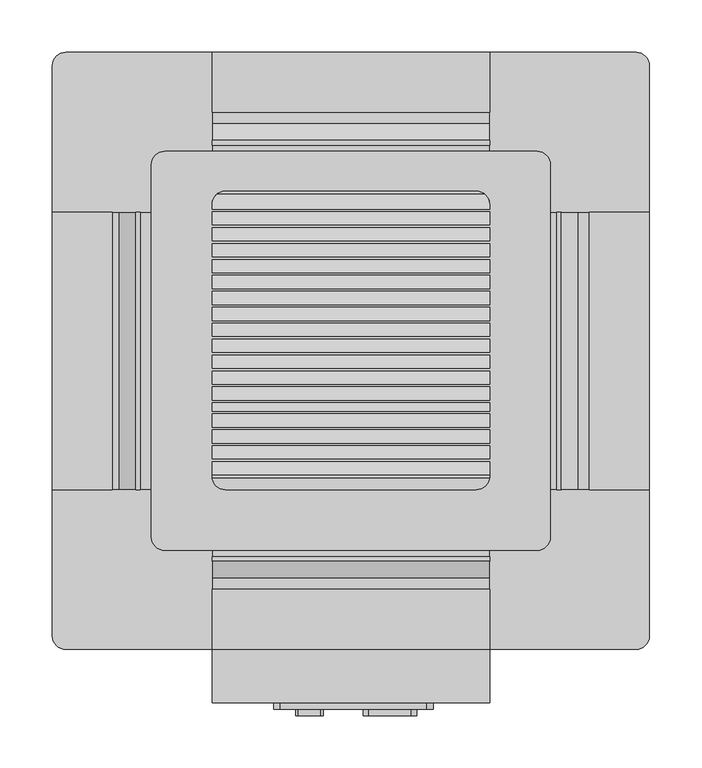
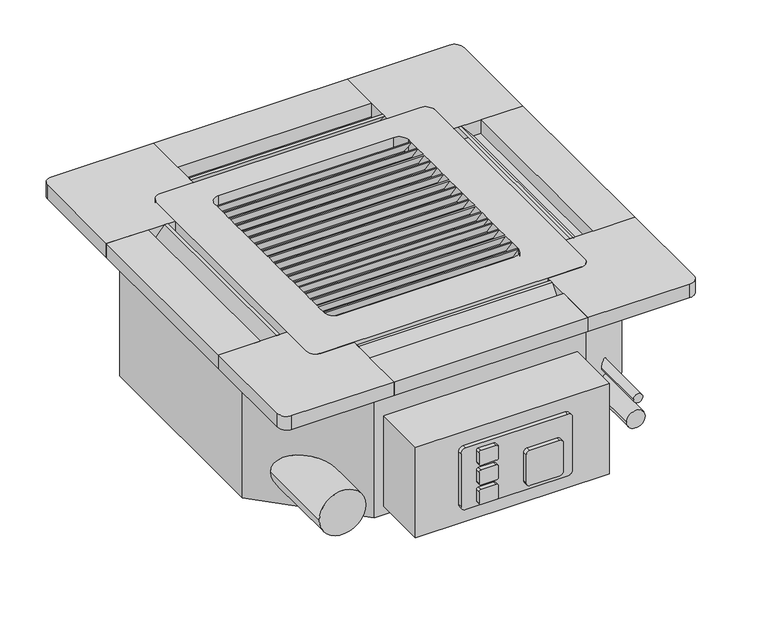
"""IFC4 building model written with IfcOpenShell, lengths in millimetres: proxy geometry, PLFY-P-NCMU-E_4-way_24x24 : PLFY-P12NCMU-E."""

import ifcopenshell
import ifcopenshell.guid

model = None  # the IFC model being written
_history = None  # IfcOwnerHistory: only IFC2X3 demands one
_inside = {}  # id of a spatial element -> (the spatial element, [elements in it])
_under = {}  # id of a project, library or spatial element -> (it, [spatial elements below it])
_declared = {}  # id of a project -> (the project, [libraries it declares])
_typed = {}  # id of a type object -> (the type object, [elements of that type])
_made_of = {}  # id of a material, layer set ... -> (it, [elements and type objects made of it])


def new_model(schema):
    """Start an empty IFC model of exactly this schema.

    Asked for "IFC4X3", IfcOpenShell would pick the latest addendum, in which some entities
    have other attributes; the version numbers below select the first issue.
    IFC2X3 requires an IfcOwnerHistory on every rooted entity: one is made here for all.
    """
    global model, _history
    if schema == "IFC4X3":
        model = ifcopenshell.file(schema_version=(4, 3, 0, 0))
    else:
        model = ifcopenshell.file(schema=schema)
    _inside.clear()
    _under.clear()
    _declared.clear()
    _typed.clear()
    _made_of.clear()
    _history = None
    if model.schema == "IFC2X3":
        org = make("IfcOrganization", Name="unknown")
        user = make(
            "IfcPersonAndOrganization",
            ThePerson=make("IfcPerson", FamilyName="unknown"),
            TheOrganization=org,
        )
        app = make(
            "IfcApplication",
            ApplicationDeveloper=org,
            Version="unknown",
            ApplicationFullName="unknown",
            ApplicationIdentifier="unknown",
        )
        _history = make(
            "IfcOwnerHistory",
            OwningUser=user,
            OwningApplication=app,
            ChangeAction="ADDED",
            CreationDate=0,
        )
    return model


def make(cls, **values):
    """One entity of the class cls with the attributes given. An attribute that is None is left unset."""
    return model.create_entity(
        cls, **{name: value for name, value in values.items() if value is not None}
    )


def rooted(cls, **values):
    """An entity with a GlobalId (a new one), such as an element, a storey or a relation."""
    return make(cls, GlobalId=ifcopenshell.guid.new(), OwnerHistory=_history, **values)


def si_unit(unit_type, name, prefix=None):
    """IfcSIUnit, for example si_unit("LENGTHUNIT", "METRE", prefix="MILLI")."""
    return make("IfcSIUnit", UnitType=unit_type, Prefix=prefix, Name=name)


def assignment(units):
    """IfcUnitAssignment: the units of a project."""
    return None if units is None else make("IfcUnitAssignment", Units=units)


def point(xyz):
    """IfcCartesianPoint."""
    return None if xyz is None else make("IfcCartesianPoint", Coordinates=xyz)


def direction(xyz):
    """IfcDirection."""
    return None if xyz is None else make("IfcDirection", DirectionRatios=xyz)


def frame(location, z_axis=None, x_axis=None):
    """IfcAxis2Placement3D, a coordinate frame: its origin and axes. An axis left out is left unset."""
    return make(
        "IfcAxis2Placement3D",
        Location=point(location),
        Axis=direction(z_axis),
        RefDirection=direction(x_axis),
    )


def frame_2d(location, x_axis=None):
    """IfcAxis2Placement2D, a coordinate frame in the plane: its origin and x axis."""
    return make(
        "IfcAxis2Placement2D", Location=point(location), RefDirection=direction(x_axis)
    )


def origin():
    """The frame at (0, 0, 0) with its axes left unset."""
    return frame((0.0, 0.0, 0.0))


def place(relative_to, where):
    """IfcLocalPlacement: puts the frame where relative to a parent placement (None: the world)."""
    return make(
        "IfcLocalPlacement", PlacementRelTo=relative_to, RelativePlacement=where
    )


def context(
    kind, dimensions, precision=None, world=None, true_north=None, identifier=None
):
    """IfcGeometricRepresentationContext, for example the 3D "Model" context."""
    return make(
        "IfcGeometricRepresentationContext",
        ContextIdentifier=identifier,
        ContextType=kind,
        CoordinateSpaceDimension=dimensions,
        Precision=precision,
        WorldCoordinateSystem=world,
        TrueNorth=true_north,
    )


def project(units=None, contexts=None):
    """IfcProject with its units and contexts."""
    return rooted(
        "IfcProject",
        Name="project",
        RepresentationContexts=contexts,
        UnitsInContext=assignment(units),
    )


def spatial(cls, under=None, at=None, **own):
    """A site, building, storey or space (cls), placed at a placement, below another one or the project."""
    s = rooted(cls, ObjectPlacement=at, **own)
    if under is not None:
        _under.setdefault(under.id(), (under, []))[1].append(s)
    return s


def polyline(points):
    """IfcPolyline through the points."""
    return make("IfcPolyline", Points=[point(p) for p in points])


def circle_curve(where, radius):
    """IfcCircle in the frame where."""
    return make("IfcCircle", Position=where, Radius=radius)


def ellipse_curve(where, semi_axis1, semi_axis2):
    """IfcEllipse in the frame where."""
    return make(
        "IfcEllipse", Position=where, SemiAxis1=semi_axis1, SemiAxis2=semi_axis2
    )


def trimmed(basis, trim1, trim2, sense, master):
    """IfcTrimmedCurve: the piece of a basis curve between two trims."""
    return make(
        "IfcTrimmedCurve",
        BasisCurve=basis,
        Trim1=trim1,
        Trim2=trim2,
        SenseAgreement=sense,
        MasterRepresentation=master,
    )


def segment(curve, same_sense, transition):
    """IfcCompositeCurveSegment."""
    return make(
        "IfcCompositeCurveSegment",
        Transition=transition,
        SameSense=same_sense,
        ParentCurve=curve,
    )


def composite_curve(segments, self_intersect=None):
    """IfcCompositeCurve: segments joined end to end."""
    return make("IfcCompositeCurve", Segments=segments, SelfIntersect=self_intersect)


def outline(outer, holes=None, kind="AREA"):
    """IfcArbitraryClosedProfileDef: a profile drawn as a closed curve; with holes, ...WithVoids."""
    if holes is None:
        return make("IfcArbitraryClosedProfileDef", ProfileType=kind, OuterCurve=outer)
    return make(
        "IfcArbitraryProfileDefWithVoids",
        ProfileType=kind,
        OuterCurve=outer,
        InnerCurves=holes,
    )


def extrude(swept, where, along, depth):
    """IfcExtrudedAreaSolid: the profile swept, set in the frame where, extruded along a direction by depth."""
    return make(
        "IfcExtrudedAreaSolid",
        SweptArea=swept,
        Position=where,
        ExtrudedDirection=direction(along),
        Depth=depth,
    )


def shape(context_of_items, identifier, shape_type, items):
    """IfcShapeRepresentation: the items that make up one representation, for example the "Body"."""
    return make(
        "IfcShapeRepresentation",
        ContextOfItems=context_of_items,
        RepresentationIdentifier=identifier,
        RepresentationType=shape_type,
        Items=items,
    )


def source(mapping_origin, context_of_items, identifier, shape_type, items):
    """IfcRepresentationMap: a shape defined once, which mapped items show again and again."""
    return make(
        "IfcRepresentationMap",
        MappingOrigin=mapping_origin,
        MappedRepresentation=shape(context_of_items, identifier, shape_type, items),
    )


def transform(
    local_origin,
    x_axis=None,
    y_axis=None,
    z_axis=None,
    scale=None,
    scale2=None,
    scale3=None,
    uniform=True,
):
    """IfcCartesianTransformationOperator3D, or its non-uniform kind. x_axis, y_axis, z_axis: its Axis1, 2, 3."""
    if uniform:
        return make(
            "IfcCartesianTransformationOperator3D",
            Axis1=direction(x_axis),
            Axis2=direction(y_axis),
            LocalOrigin=point(local_origin),
            Scale=scale,
            Axis3=direction(z_axis),
        )
    return make(
        "IfcCartesianTransformationOperator3DnonUniform",
        Axis1=direction(x_axis),
        Axis2=direction(y_axis),
        LocalOrigin=point(local_origin),
        Scale=scale,
        Axis3=direction(z_axis),
        Scale2=scale2,
        Scale3=scale3,
    )


def mapped(mapping_source, mapping_target):
    """IfcMappedItem: shows the shape of a source again, moved by a transform."""
    return make(
        "IfcMappedItem", MappingSource=mapping_source, MappingTarget=mapping_target
    )


def made_of(thing, what):
    """Note that an element or type object is made of a material, layer set ...; save() writes the relation."""
    if what is not None:
        _made_of.setdefault(what.id(), (what, []))[1].append(thing)
    return thing


def element(
    cls,
    number,
    at=None,
    inside=None,
    cuts=None,
    type_object=None,
    material=None,
    context=None,
    identifier="Body",
    shape_type=None,
    held_by="IfcProductDefinitionShape",
    body=None,
    shapes=None,
    **own,
):
    """One element of the class cls, such as IfcWall. Its Tag is "e" and its number.

    at: its placement. inside: the storey or other place that contains it. cuts: it is an
    opening in that element (IfcRelVoidsElement). A single representation is given by context,
    identifier, shape_type and body (its items); several are given by shapes. held_by: the class
    of the entity that holds the representations. save() writes the other relations.
    """
    e = rooted(cls, Tag="e%d" % number, ObjectPlacement=at, **own)
    if body is not None:
        shapes = [shape(context, identifier, shape_type, body)]
    if shapes is not None:
        e.Representation = make(held_by, Representations=shapes)
    if inside is not None:
        _inside.setdefault(inside.id(), (inside, []))[1].append(e)
    if cuts is not None:
        rooted(
            "IfcRelVoidsElement", RelatingBuildingElement=cuts, RelatedOpeningElement=e
        )
    if type_object is not None:
        _typed.setdefault(type_object.id(), (type_object, []))[1].append(e)
    return made_of(e, material)


def aggregate(whole, parts):
    """IfcRelAggregates: a whole, such as a stair, and the parts it consists of."""
    return rooted("IfcRelAggregates", RelatingObject=whole, RelatedObjects=parts)


def save(model, path):
    """Write the relations noted so far, then the file.

    IfcRelAggregates (storeys below a building ...), IfcRelContainedInSpatialStructure (elements
    in a storey), IfcRelDefinesByType, IfcRelAssociatesMaterial and IfcRelDeclares: one each for
    every whole, place, type object, material and project.
    """
    for whole, parts in _under.values():
        aggregate(whole, parts)
    for where, things in _inside.values():
        rooted(
            "IfcRelContainedInSpatialStructure",
            RelatedElements=things,
            RelatingStructure=where,
        )
    for kind, things in _typed.values():
        rooted("IfcRelDefinesByType", RelatedObjects=things, RelatingType=kind)
    for what, things in _made_of.values():
        rooted("IfcRelAssociatesMaterial", RelatedObjects=things, RelatingMaterial=what)
    for by, libraries in _declared.values():
        rooted("IfcRelDeclares", RelatingContext=by, RelatedDefinitions=libraries)
    model.write(path)


def plane_surface(at):
    """IfcPlane: the flat surface through the origin of the frame at, square to its z axis."""
    return make("IfcPlane", Position=at)


def cylinder_surface(at, radius):
    """IfcCylindricalSurface: all points at the distance radius from the z axis of the frame at."""
    return make("IfcCylindricalSurface", Position=at, Radius=radius)


def revolved_surface(curve, axis_point, axis_direction):
    """IfcSurfaceOfRevolution: the curve turned about the line through axis_point along axis_direction."""
    return make(
        "IfcSurfaceOfRevolution",
        SweptCurve=make("IfcArbitraryOpenProfileDef", ProfileType="CURVE", Curve=curve),
        AxisPosition=make("IfcAxis1Placement", Location=point(axis_point), Axis=direction(axis_direction)),
    )


def advanced_brep(points, edges, surfaces, faces):
    """IfcAdvancedBrep: a solid bounded by faces that lie on surfaces and meet in shared edges.

    An edge is (start, end): straight between two places in points (the first is 0);
    or (start, end, curve); or (start, end, curve, False) where it runs against its curve.
    A face is (place in surfaces, loops), or (place, loops, False) where it looks against
    its surface's normal. A loop lists edges by number (the first is 1), with a minus sign
    where the edge is run from its end to its start. The first loop is the outer one.
    """
    corners = [point(p) for p in points]
    vertices = [make("IfcVertexPoint", VertexGeometry=c) for c in corners]
    made = []
    for start, end, *more in edges:
        made.append(
            make(
                "IfcEdgeCurve",
                EdgeStart=vertices[start],
                EdgeEnd=vertices[end],
                EdgeGeometry=more[0] if more else make("IfcPolyline", Points=[corners[start], corners[end]]),
                SameSense=more[1] if len(more) > 1 else True,
            )
        )
    hull = []
    for where, loops, *sense in faces:
        bounds = []
        for j, loop in enumerate(loops):
            ring = [make("IfcOrientedEdge", EdgeElement=made[abs(k) - 1], Orientation=k > 0) for k in loop]
            bounds.append(
                make(
                    "IfcFaceOuterBound" if j == 0 else "IfcFaceBound",
                    Bound=make("IfcEdgeLoop", EdgeList=ring),
                    Orientation=True,
                )
            )
        hull.append(make("IfcAdvancedFace", Bounds=bounds, FaceSurface=surfaces[where], SameSense=sense[0] if sense else True))
    return make("IfcAdvancedBrep", Outer=make("IfcClosedShell", CfsFaces=hull))


def mechanical_equipment_2d84379e(model_context):
    return source(origin(), model_context, "Body", "SolidModel", [
        extrude(outline(polyline([(284.95625, -201.1772913), (227.80625, -201.1772913), (227.80625, 63.9352087), (284.95625, 63.9352087), (284.95625, -201.1772913)])), frame((0.0, 0.0, -1.02e-05), z_axis=(0.0, 0.0, 1.0), x_axis=(1.0, 0.0, 0.0)), (0.0, 0.0, 1.0), 19.84375),
        extrude(outline(polyline([(-284.95625, -201.1772913), (-284.95625, 63.9352087), (-227.80625, 63.9352087), (-227.80625, -201.1772913), (-284.95625, -201.1772913)])), frame((0.0, 0.0, -1.02e-05), z_axis=(0.0, 0.0, 1.0), x_axis=(1.0, 0.0, 0.0)), (0.0, 0.0, 1.0), 19.84375),
        extrude(outline(polyline([(-132.55625, 216.3352087), (132.55625, 216.3352087), (132.55625, 159.1852087), (-132.55625, 159.1852087), (-132.55625, 216.3352087)])), frame((0.0, 0.0, -1.02e-05), z_axis=(0.0, 0.0, 1.0), x_axis=(1.0, 0.0, 0.0)), (0.0, 0.0, 1.0), 19.84375),
        extrude(outline(polyline([(-132.55625, -353.5772913), (-132.55625, -296.4272913), (132.55625, -296.4272913), (132.55625, -353.5772913), (-132.55625, -353.5772913)])), frame((0.0, 0.0, -1.02e-05), z_axis=(0.0, 0.0, 1.0), x_axis=(1.0, 0.0, 0.0)), (0.0, 0.0, 1.0), 19.84375),
        extrude(outline(polyline([(-187.079491, 19.8437398), (-173.1847477, -1.02e-05), (-175.7772913, -1.02e-05), (-189.6720346, 19.8437398), (-187.079491, 19.8437398)])), frame((-132.55625, 0.0, 0.0), z_axis=(1.0, 0.0, 0.0), x_axis=(0.0, 1.0, 0.0)), (0.0, 0.0, 1.0), 265.1125),
        advanced_brep(
        [(-177.8, -259.1210413, -1.02e-05), (-190.5, -246.4210413, -1.02e-05), (-190.5, 109.1789587, -1.02e-05), (-177.8, 121.8789587, -1.02e-05), (177.8, 121.8789587, -1.02e-05), (190.5, 109.1789587, -1.02e-05), (190.5, -246.4210413, -1.02e-05), (177.8, -259.1210413, -1.02e-05), (132.55625, -130.1575084, -1.02e-05), (-132.55625, -130.1575084, -1.02e-05), (-132.55625, -142.7715591, -1.02e-05), (132.55625, -142.7715591, -1.02e-05), (132.55625, -114.9509141, -1.02e-05), (-132.55625, -114.9509141, -1.02e-05), (-132.55625, -127.5649648, -1.02e-05), (132.55625, -127.5649648, -1.02e-05), (132.55625, -104.3814755, -1.02e-05), (-132.55625, -104.3814755, -1.02e-05), (-132.55625, -112.3583705, -1.02e-05), (132.55625, -112.3583705, -1.02e-05), (132.55625, -89.1748812, -1.02e-05), (-132.55625, -89.1748812, -1.02e-05), (-132.55625, -101.7889319, -1.02e-05), (132.55625, -101.7889319, -1.02e-05), (132.55625, -73.9682869, -1.02e-05), (-132.55625, -73.9682869, -1.02e-05), (-132.55625, -86.5823376, -1.02e-05), (132.55625, -86.5823376, -1.02e-05), (132.55625, -58.7616926, -1.02e-05), (-132.55625, -58.7616926, -1.02e-05), (-132.55625, -71.3757433, -1.02e-05), (132.55625, -71.3757433, -1.02e-05), (132.55625, -43.5550983, -1.02e-05), (-132.55625, -43.5550983, -1.02e-05), (-132.55625, -56.169149, -1.02e-05), (132.55625, -56.169149, -1.02e-05), (132.55625, -28.348504, -1.02e-05), (-132.55625, -28.348504, -1.02e-05), (-132.55625, -40.9625547, -1.02e-05), (132.55625, -40.9625547, -1.02e-05), (132.55625, -13.1419097, -1.02e-05), (-132.55625, -13.1419097, -1.02e-05), (-132.55625, -25.7559604, -1.02e-05), (132.55625, -25.7559604, -1.02e-05), (132.55625, 32.4778732, -1.02e-05), (-132.55625, 32.4778732, -1.02e-05), (-132.55625, 19.8638225, -1.02e-05), (132.55625, 19.8638225, -1.02e-05), (132.55625, 47.6844675, -1.02e-05), (-132.55625, 47.6844675, -1.02e-05), (-132.55625, 35.0704168, -1.02e-05), (132.55625, 35.0704168, -1.02e-05), (132.55625, 62.8910618, -1.02e-05), (-132.55625, 62.8910618, -1.02e-05), (-132.55625, 50.2770111, -1.02e-05), (132.55625, 50.2770111, -1.02e-05), (132.55625, 2.0646846, -1.02e-05), (-132.55625, 2.0646846, -1.02e-05), (-132.55625, -10.5493661, -1.02e-05), (132.55625, -10.5493661, -1.02e-05), (-132.55625, 4.6572282, -1.02e-05), (132.55625, 4.6572282, -1.02e-05), (132.55625, 17.2712789, -1.02e-05), (-132.55625, 17.2712789, -1.02e-05), (132.55625, 71.0789587, -1.02e-05), (130.4405727, 78.0976561, -1.02e-05), (-130.4405727, 78.0976561, -1.02e-05), (-132.55625, 71.0789587, -1.02e-05), (-132.55625, 65.4836054, -1.02e-05), (132.55625, 65.4836054, -1.02e-05), (-132.55625, -145.3641027, -1.02e-05), (-132.55625, -157.9781534, -1.02e-05), (132.55625, -157.9781534, -1.02e-05), (132.55625, -145.3641027, -1.02e-05), (-132.55625, -188.4772913, -1.02e-05), (-119.85625, -201.1772913, -1.02e-05), (119.85625, -201.1772913, -1.02e-05), (132.55625, -188.4772913, -1.02e-05), (132.55625, -160.570697, -1.02e-05), (-132.55625, -160.570697, -1.02e-05), (119.85625, 83.7789587, -1.02e-05), (-119.85625, 83.7789587, -1.02e-05), (-128.1576984, 80.6901997, -1.02e-05), (128.1576984, 80.6901997, -1.02e-05), (-177.8, -259.1210413, 19.8437398), (177.8, -259.1210413, 19.8437398), (190.5, -246.4210413, 19.8437398), (190.5, 109.1789587, 19.8437398), (177.8, 121.8789587, 19.8437398), (-177.8, 121.8789587, 19.8437398), (-190.5, 109.1789587, 19.8437398), (-190.5, -246.4210413, 19.8437398), (-132.55625, -144.0522517, 19.8437398), (132.55625, -144.0522517, 19.8437398), (132.55625, -156.6663024, 19.8437398), (-132.55625, -156.6663024, 19.8437398), (-132.55625, -128.8456574, 19.8437398), (132.55625, -128.8456574, 19.8437398), (132.55625, -141.4597081, 19.8437398), (-132.55625, -141.4597081, 19.8437398), (-132.55625, -118.2762188, 19.8437398), (132.55625, -118.2762188, 19.8437398), (132.55625, -126.2531138, 19.8437398), (-132.55625, -126.2531138, 19.8437398), (-132.55625, -103.0696245, 19.8437398), (132.55625, -103.0696245, 19.8437398), (132.55625, -115.6836752, 19.8437398), (-132.55625, -115.6836752, 19.8437398), (-132.55625, -87.8630302, 19.8437398), (132.55625, -87.8630302, 19.8437398), (132.55625, -100.4770809, 19.8437398), (-132.55625, -100.4770809, 19.8437398), (-132.55625, -72.6564359, 19.8437398), (132.55625, -72.6564359, 19.8437398), (132.55625, -85.2704866, 19.8437398), (-132.55625, -85.2704866, 19.8437398), (-132.55625, -57.4498416, 19.8437398), (132.55625, -57.4498416, 19.8437398), (132.55625, -70.0638923, 19.8437398), (-132.55625, -70.0638923, 19.8437398), (-132.55625, -42.2432473, 19.8437398), (132.55625, -42.2432473, 19.8437398), (132.55625, -54.857298, 19.8437398), (-132.55625, -54.857298, 19.8437398), (-132.55625, -27.036653, 19.8437398), (132.55625, -27.036653, 19.8437398), (132.55625, -39.6507037, 19.8437398), (-132.55625, -39.6507037, 19.8437398), (-132.55625, 18.5831298, 19.8437398), (132.55625, 18.5831298, 19.8437398), (132.55625, 5.9690792, 19.8437398), (-132.55625, 5.9690792, 19.8437398), (-132.55625, 33.7897241, 19.8437398), (132.55625, 33.7897241, 19.8437398), (132.55625, 21.1756735, 19.8437398), (-132.55625, 21.1756735, 19.8437398), (-132.55625, 48.9963184, 19.8437398), (132.55625, 48.9963184, 19.8437398), (132.55625, 36.3822678, 19.8437398), (-132.55625, 36.3822678, 19.8437398), (-132.55625, -11.8300587, 19.8437398), (132.55625, -11.8300587, 19.8437398), (132.55625, -24.4441094, 19.8437398), (-132.55625, -24.4441094, 19.8437398), (132.55625, -9.2375151, 19.8437398), (-132.55625, -9.2375151, 19.8437398), (-132.55625, 3.3765356, 19.8437398), (132.55625, 3.3765356, 19.8437398), (-132.55625, 64.2029127, 19.8437398), (132.55625, 64.2029127, 19.8437398), (132.55625, 51.5888621, 19.8437398), (-132.55625, 51.5888621, 19.8437398), (-132.55625, 71.0789587, 19.8437398), (-119.85625, 83.7789587, 19.8437398), (119.85625, 83.7789587, 19.8437398), (132.55625, 71.0789587, 19.8437398), (132.55625, 66.7954564, 19.8437398), (-132.55625, 66.7954564, 19.8437398), (132.55625, -159.258846, 19.8437398), (132.55625, -171.8728967, 19.8437398), (-132.55625, -171.8728967, 19.8437398), (-132.55625, -159.258846, 19.8437398), (132.55625, -188.4772913, 19.8437398), (119.85625, -201.1772913, 19.8437398), (-119.85625, -201.1772913, 19.8437398), (-132.55625, -188.4772913, 19.8437398), (-132.55625, -174.4654403, 19.8437398), (132.55625, -174.4654403, 19.8437398), (132.55625, 71.0789587, 13.7262645), (132.55625, 71.0789587, 10.0237284), (-132.55625, 71.0789587, 10.0237284), (-132.55625, 71.0789587, 13.7262645)],
        [
            (0, 1, circle_curve(frame((-177.8, -246.4210413, -1.02e-05), z_axis=(0.0, 0.0, -1.0), x_axis=(-1.0, 0.0, 0.0)), 12.7)),
            (1, 2),
            (2, 3, circle_curve(frame((-177.8, 109.1789587, -1.02e-05), z_axis=(0.0, 0.0, -1.0), x_axis=(-1.0, 0.0, 0.0)), 12.7)),
            (3, 4),
            (4, 5, circle_curve(frame((177.8, 109.1789587, -1.02e-05), z_axis=(0.0, 0.0, -1.0), x_axis=(-1.0, 0.0, 0.0)), 12.7)),
            (5, 6),
            (6, 7, circle_curve(frame((177.8, -246.4210413, -1.02e-05), z_axis=(0.0, 0.0, -1.0), x_axis=(-1.0, 0.0, 0.0)), 12.7)),
            (7, 0),
            (8, 9),
            (9, 10),
            (10, 11),
            (11, 8),
            (12, 13),
            (13, 14),
            (14, 15),
            (15, 12),
            (16, 17),
            (17, 18),
            (18, 19),
            (19, 16),
            (20, 21),
            (21, 22),
            (22, 23),
            (23, 20),
            (24, 25),
            (25, 26),
            (26, 27),
            (27, 24),
            (28, 29),
            (29, 30),
            (30, 31),
            (31, 28),
            (32, 33),
            (33, 34),
            (34, 35),
            (35, 32),
            (36, 37),
            (37, 38),
            (38, 39),
            (39, 36),
            (40, 41),
            (41, 42),
            (42, 43),
            (43, 40),
            (44, 45),
            (45, 46),
            (46, 47),
            (47, 44),
            (48, 49),
            (49, 50),
            (50, 51),
            (51, 48),
            (52, 53),
            (53, 54),
            (54, 55),
            (55, 52),
            (56, 57),
            (57, 58),
            (58, 59),
            (59, 56),
            (60, 61),
            (61, 62),
            (62, 63),
            (63, 60),
            (64, 65, circle_curve(frame((119.85625, 71.0789587, -1.02e-05), z_axis=(0.0, 0.0, 1.0), x_axis=(-1.0, 0.0, 0.0)), 12.7)),
            (65, 66),
            (66, 67, circle_curve(frame((-119.85625, 71.0789587, -1.02e-05), z_axis=(0.0, 0.0, 1.0), x_axis=(-1.0, 0.0, 0.0)), 12.7)),
            (67, 68),
            (68, 69),
            (69, 64),
            (70, 71),
            (71, 72),
            (72, 73),
            (73, 70),
            (74, 75, circle_curve(frame((-119.85625, -188.4772913, -1.02e-05), z_axis=(0.0, 0.0, 1.0), x_axis=(-1.0, 0.0, 0.0)), 12.7)),
            (75, 76),
            (76, 77, circle_curve(frame((119.85625, -188.4772913, -1.02e-05), z_axis=(0.0, 0.0, 1.0), x_axis=(-1.0, 0.0, 0.0)), 12.7)),
            (77, 78),
            (78, 79),
            (79, 74),
            (80, 81),
            (81, 82, circle_curve(frame((-119.85625, 71.0789587, -1.02e-05), z_axis=(0.0, 0.0, 1.0), x_axis=(-1.0, 0.0, 0.0)), 12.7)),
            (82, 83),
            (83, 80, circle_curve(frame((119.85625, 71.0789587, -1.02e-05), z_axis=(0.0, 0.0, 1.0), x_axis=(-1.0, 0.0, 0.0)), 12.7)),
            (84, 85),
            (85, 86, circle_curve(frame((177.8, -246.4210413, 19.8437398), z_axis=(0.0, 0.0, 1.0), x_axis=(-1.0, 0.0, 0.0)), 12.7)),
            (86, 87),
            (87, 88, circle_curve(frame((177.8, 109.1789587, 19.8437398), z_axis=(0.0, 0.0, 1.0), x_axis=(-1.0, 0.0, 0.0)), 12.7)),
            (88, 89),
            (89, 90, circle_curve(frame((-177.8, 109.1789587, 19.8437398), z_axis=(0.0, 0.0, 1.0), x_axis=(-1.0, 0.0, 0.0)), 12.7)),
            (90, 91),
            (91, 84, circle_curve(frame((-177.8, -246.4210413, 19.8437398), z_axis=(0.0, 0.0, 1.0), x_axis=(-1.0, 0.0, 0.0)), 12.7)),
            (92, 93),
            (93, 94),
            (94, 95),
            (95, 92),
            (96, 97),
            (97, 98),
            (98, 99),
            (99, 96),
            (100, 101),
            (101, 102),
            (102, 103),
            (103, 100),
            (104, 105),
            (105, 106),
            (106, 107),
            (107, 104),
            (108, 109),
            (109, 110),
            (110, 111),
            (111, 108),
            (112, 113),
            (113, 114),
            (114, 115),
            (115, 112),
            (116, 117),
            (117, 118),
            (118, 119),
            (119, 116),
            (120, 121),
            (121, 122),
            (122, 123),
            (123, 120),
            (124, 125),
            (125, 126),
            (126, 127),
            (127, 124),
            (128, 129),
            (129, 130),
            (130, 131),
            (131, 128),
            (132, 133),
            (133, 134),
            (134, 135),
            (135, 132),
            (136, 137),
            (137, 138),
            (138, 139),
            (139, 136),
            (140, 141),
            (141, 142),
            (142, 143),
            (143, 140),
            (144, 145),
            (145, 146),
            (146, 147),
            (147, 144),
            (148, 149),
            (149, 150),
            (150, 151),
            (151, 148),
            (152, 153, circle_curve(frame((-119.85625, 71.0789587, 19.8437398), z_axis=(0.0, 0.0, -1.0), x_axis=(-1.0, 0.0, 0.0)), 12.7)),
            (153, 154),
            (154, 155, circle_curve(frame((119.85625, 71.0789587, 19.8437398), z_axis=(0.0, 0.0, -1.0), x_axis=(-1.0, 0.0, 0.0)), 12.7)),
            (155, 156),
            (156, 157),
            (157, 152),
            (158, 159),
            (159, 160),
            (160, 161),
            (161, 158),
            (162, 163, circle_curve(frame((119.85625, -188.4772913, 19.8437398), z_axis=(0.0, 0.0, -1.0), x_axis=(-1.0, 0.0, 0.0)), 12.7)),
            (163, 164),
            (164, 165, circle_curve(frame((-119.85625, -188.4772913, 19.8437398), z_axis=(0.0, 0.0, -1.0), x_axis=(-1.0, 0.0, 0.0)), 12.7)),
            (165, 166),
            (166, 167),
            (167, 162),
            (155, 168),
            (168, 156),
            (77, 162),
            (167, 78),
            (169, 64),
            (69, 150),
            (149, 169),
            (61, 144),
            (147, 62),
            (141, 56),
            (59, 142),
            (137, 52),
            (55, 138),
            (133, 48),
            (51, 134),
            (129, 44),
            (47, 130),
            (125, 40),
            (43, 126),
            (121, 36),
            (39, 122),
            (117, 32),
            (35, 118),
            (113, 28),
            (31, 114),
            (109, 24),
            (27, 110),
            (105, 20),
            (23, 106),
            (101, 16),
            (19, 102),
            (97, 12),
            (15, 98),
            (93, 8),
            (11, 94),
            (158, 73),
            (72, 159),
            (169, 65, ellipse_curve(frame((119.85625, 71.0789587, 10.0237284), z_axis=(0.0, 0.8191520442889908, 0.5735764363510476), x_axis=(0.0, -0.5735764363510477, 0.8191520442889908)), 22.1417743, 12.7)),
            (154, 80),
            (83, 168, ellipse_curve(frame((119.85625, 71.0789587, 13.7262645), z_axis=(0.0, -0.8191520442889919, -0.573576436351046), x_axis=(0.0, -0.5735764363510462, 0.8191520442889919)), 22.1417743, 12.7)),
            (153, 81),
            (66, 170, ellipse_curve(frame((-119.85625, 71.0789587, 10.0237284), z_axis=(0.0, 0.8191520442889908, 0.5735764363510476), x_axis=(0.0, -0.5735764363510477, 0.8191520442889908)), 22.1417743, 12.7)),
            (170, 67),
            (152, 171),
            (171, 82, ellipse_curve(frame((-119.85625, 71.0789587, 13.7262645), z_axis=(0.0, -0.8191520442889919, -0.573576436351046), x_axis=(0.0, -0.5735764363510462, 0.8191520442889919)), 22.1417743, 12.7)),
            (157, 171),
            (170, 148),
            (151, 68),
            (165, 74),
            (79, 166),
            (145, 60),
            (63, 146),
            (57, 140),
            (143, 58),
            (53, 136),
            (139, 54),
            (49, 132),
            (135, 50),
            (45, 128),
            (131, 46),
            (41, 124),
            (127, 42),
            (37, 120),
            (123, 38),
            (33, 116),
            (119, 34),
            (29, 112),
            (115, 30),
            (25, 108),
            (111, 26),
            (21, 104),
            (107, 22),
            (17, 100),
            (103, 18),
            (13, 96),
            (99, 14),
            (9, 92),
            (95, 10),
            (70, 161),
            (160, 71),
            (164, 75),
            (163, 76),
            (0, 84),
            (91, 1),
            (90, 2),
            (89, 3),
            (88, 4),
            (87, 5),
            (86, 6),
            (85, 7),
        ],
        [
            plane_surface(frame((132.55625, 71.0789587, -1.02e-05), z_axis=(0.0, 0.0, -1.0), x_axis=(0.0, 1.0, 0.0))),
            plane_surface(frame((132.55625, 71.0789587, 19.8437398), z_axis=(0.0, 0.0, 1.0), x_axis=(0.0, -1.0, 0.0))),
            plane_surface(frame((132.55625, -188.4772913, -1.02e-05), z_axis=(-1.0, 0.0, 0.0), x_axis=(0.0, 0.0, 1.0))),
            revolved_surface(polyline([(107.15625, 71.0789587, 28.161208082030438), (107.15625, 71.0789587, -8.113751282030439)]), (119.85625, 71.0789587, 19.8437398), (0.0, 0.0, 1.0)),
            revolved_surface(polyline([(107.15625, 71.0789587, 31.863744182030462), (107.15625, 71.0789587, -4.411215182030464)]), (119.85625, 71.0789587, 19.8437398), (0.0, 0.0, 1.0)),
            plane_surface(frame((119.85625, 83.7789587, -1.02e-05), z_axis=(0.0, -1.0, 0.0), x_axis=(0.0, 0.0, 1.0))),
            revolved_surface(polyline([(-132.55625, 71.0789587, 28.161208082030438), (-132.55625, 71.0789587, -8.113751282030439)]), (-119.85625, 71.0789587, 19.8437398), (0.0, 0.0, 1.0)),
            revolved_surface(polyline([(-132.55625, 71.0789587, 31.863744182030462), (-132.55625, 71.0789587, -4.411215182030464)]), (-119.85625, 71.0789587, 19.8437398), (0.0, 0.0, 1.0)),
            plane_surface(frame((-132.55625, 71.0789587, -1.02e-05), z_axis=(1.0, 0.0, 0.0), x_axis=(0.0, 0.0, 1.0))),
            revolved_surface(polyline([(-132.55625, -188.4772913, 19.8437398), (-132.55625, -188.4772913, -1.0199999998405929e-05)]), (-119.85625, -188.4772913, 19.8437398), (0.0, 0.0, 1.0)),
            plane_surface(frame((-119.85625, -201.1772913, -1.02e-05), z_axis=(0.0, 1.0, 0.0), x_axis=(0.0, 0.0, 1.0))),
            revolved_surface(polyline([(107.15625, -188.4772913, 19.8437398), (107.15625, -188.4772913, -1.0199999998405929e-05)]), (119.85625, -188.4772913, 19.8437398), (0.0, 0.0, 1.0)),
            cylinder_surface(frame((-177.8, -246.4210413, -1.02e-05), z_axis=(0.0, 0.0, -1.0), x_axis=(-1.0, 0.0, 0.0)), 12.7),
            plane_surface(frame((-190.5, -246.4210413, -1.02e-05), z_axis=(-1.0, 0.0, 0.0), x_axis=(0.0, 0.0, 1.0))),
            cylinder_surface(frame((-177.8, 109.1789587, -1.02e-05), z_axis=(0.0, 0.0, -1.0), x_axis=(-1.0, 0.0, 0.0)), 12.7),
            plane_surface(frame((-177.8, 121.8789587, -1.02e-05), z_axis=(0.0, 1.0, 0.0), x_axis=(0.0, 0.0, 1.0))),
            cylinder_surface(frame((177.8, 109.1789587, -1.02e-05), z_axis=(0.0, 0.0, -1.0), x_axis=(-1.0, 0.0, 0.0)), 12.7),
            plane_surface(frame((190.5, 109.1789587, -1.02e-05), z_axis=(1.0, 0.0, 0.0), x_axis=(0.0, 0.0, 1.0))),
            cylinder_surface(frame((177.8, -246.4210413, -1.02e-05), z_axis=(0.0, 0.0, -1.0), x_axis=(-1.0, 0.0, 0.0)), 12.7),
            plane_surface(frame((177.8, -259.1210413, -1.02e-05), z_axis=(0.0, -1.0, 0.0), x_axis=(0.0, 0.0, 1.0))),
            plane_surface(frame((-132.55625, 66.7954564, 19.8437398), z_axis=(0.0, 0.8191520442889919, 0.573576436351046), x_axis=(1.0, 0.0, 0.0))),
            plane_surface(frame((-132.55625, 78.0976561, -1.02e-05), z_axis=(0.0, -0.8191520442889908, -0.5735764363510476), x_axis=(1.0, 0.0, 0.0))),
            plane_surface(frame((-132.55625, -9.2375151, 19.8437398), z_axis=(0.0, 0.8191520442889919, 0.573576436351046), x_axis=(1.0, 0.0, 0.0))),
            plane_surface(frame((-132.55625, 2.0646846, -1.02e-05), z_axis=(0.0, -0.8191520442889908, -0.5735764363510476), x_axis=(1.0, 0.0, 0.0))),
            plane_surface(frame((-132.55625, 51.5888621, 19.8437398), z_axis=(0.0, 0.8191520442889909, 0.5735764363510475), x_axis=(1.0, 0.0, 0.0))),
            plane_surface(frame((-132.55625, 62.8910618, -1.02e-05), z_axis=(0.0, -0.8191520442889917, -0.5735764363510462), x_axis=(1.0, 0.0, 0.0))),
            plane_surface(frame((-132.55625, 36.3822678, 19.8437398), z_axis=(0.0, 0.8191520442889899, 0.5735764363510489), x_axis=(1.0, 0.0, 0.0))),
            plane_surface(frame((-132.55625, 47.6844675, -1.02e-05), z_axis=(0.0, -0.8191520442889901, -0.5735764363510485), x_axis=(1.0, 0.0, 0.0))),
            plane_surface(frame((-132.55625, 21.1756735, 19.8437398), z_axis=(0.0, 0.8191520442889908, 0.5735764363510477), x_axis=(1.0, 0.0, 0.0))),
            plane_surface(frame((-132.55625, 32.4778732, -1.02e-05), z_axis=(0.0, -0.8191520442889919, -0.5735764363510462), x_axis=(1.0, 0.0, 0.0))),
            plane_surface(frame((-132.55625, 5.9690792, 19.8437398), z_axis=(0.0, 0.8191520442889905, 0.5735764363510482), x_axis=(1.0, 0.0, 0.0))),
            plane_surface(frame((-132.55625, 17.2712789, -1.02e-05), z_axis=(0.0, -0.8191520442889922, -0.5735764363510455), x_axis=(1.0, 0.0, 0.0))),
            plane_surface(frame((-132.55625, -24.4441094, 19.8437398), z_axis=(0.0, 0.8191520442889909, 0.5735764363510475), x_axis=(1.0, 0.0, 0.0))),
            plane_surface(frame((-132.55625, -13.1419097, -1.02e-05), z_axis=(0.0, -0.8191520442889917, -0.5735764363510462), x_axis=(1.0, 0.0, 0.0))),
            plane_surface(frame((-132.55625, -39.6507037, 19.8437398), z_axis=(0.0, 0.8191520442889902, 0.5735764363510484), x_axis=(1.0, 0.0, 0.0))),
            plane_surface(frame((-132.55625, -28.348504, -1.02e-05), z_axis=(0.0, -0.8191520442889924, -0.5735764363510453), x_axis=(1.0, 0.0, 0.0))),
            plane_surface(frame((-132.55625, -54.857298, 19.8437398), z_axis=(0.0, 0.8191520442889916, 0.5735764363510465), x_axis=(1.0, 0.0, 0.0))),
            plane_surface(frame((-132.55625, -43.5550983, -1.02e-05), z_axis=(0.0, -0.8191520442889911, -0.5735764363510472), x_axis=(1.0, 0.0, 0.0))),
            plane_surface(frame((-132.55625, -70.0638923, 19.8437398), z_axis=(0.0, 0.8191520442889899, 0.5735764363510489), x_axis=(1.0, 0.0, 0.0))),
            plane_surface(frame((-132.55625, -58.7616926, -1.02e-05), z_axis=(0.0, -0.8191520442889901, -0.5735764363510485), x_axis=(1.0, 0.0, 0.0))),
            plane_surface(frame((-132.55625, -85.2704866, 19.8437398), z_axis=(0.0, 0.8191520442889914, 0.5735764363510468), x_axis=(1.0, 0.0, 0.0))),
            plane_surface(frame((-132.55625, -73.9682869, -1.02e-05), z_axis=(0.0, -0.8191520442889915, -0.5735764363510467), x_axis=(1.0, 0.0, 0.0))),
            plane_surface(frame((-132.55625, -100.4770809, 19.8437398), z_axis=(0.0, 0.8191520442889907, 0.5735764363510477), x_axis=(1.0, 0.0, 0.0))),
            plane_surface(frame((-132.55625, -89.1748812, -1.02e-05), z_axis=(0.0, -0.8191520442889921, -0.5735764363510457), x_axis=(1.0, 0.0, 0.0))),
            plane_surface(frame((-132.55625, -115.6836752, 19.8437398), z_axis=(0.0, 0.819152044288992, 0.5735764363510459), x_axis=(1.0, 0.0, 0.0))),
            plane_surface(frame((-132.55625, -104.3814755, -1.02e-05), z_axis=(0.0, -0.8191520442889908, -0.5735764363510476), x_axis=(1.0, 0.0, 0.0))),
            plane_surface(frame((-132.55625, -126.2531138, 19.8437398), z_axis=(0.0, 0.8191520442889881, 0.5735764363510515), x_axis=(1.0, 0.0, 0.0))),
            plane_surface(frame((-132.55625, -114.9509141, -1.02e-05), z_axis=(0.0, -0.8191520442889907, -0.5735764363510477), x_axis=(1.0, 0.0, 0.0))),
            plane_surface(frame((-132.55625, -141.4597081, 19.8437398), z_axis=(0.0, 0.8191520442889891, 0.5735764363510499), x_axis=(1.0, 0.0, 0.0))),
            plane_surface(frame((-132.55625, -130.1575084, -1.02e-05), z_axis=(0.0, -0.819152044288991, -0.5735764363510474), x_axis=(1.0, 0.0, 0.0))),
            plane_surface(frame((-132.55625, -156.6663024, 19.8437398), z_axis=(0.0, 0.8191520442889885, 0.5735764363510508), x_axis=(1.0, 0.0, 0.0))),
            plane_surface(frame((-132.55625, -145.3641027, -1.02e-05), z_axis=(0.0, -0.819152044288991, -0.5735764363510474), x_axis=(1.0, 0.0, 0.0))),
            plane_surface(frame((-132.55625, -171.8728967, 19.8437398), z_axis=(0.0, 0.8191520442889885, 0.5735764363510508), x_axis=(1.0, 0.0, 0.0))),
            plane_surface(frame((-132.55625, -160.570697, -1.02e-05), z_axis=(0.0, -0.819152044288991, -0.5735764363510474), x_axis=(1.0, 0.0, 0.0))),
        ],
        [
            (0, [[1, 2, 3, 4, 5, 6, 7, 8], [9, 10, 11, 12], [13, 14, 15, 16], [17, 18, 19, 20], [21, 22, 23, 24], [25, 26, 27, 28], [29, 30, 31, 32], [33, 34, 35, 36], [37, 38, 39, 40], [41, 42, 43, 44], [45, 46, 47, 48], [49, 50, 51, 52], [53, 54, 55, 56], [57, 58, 59, 60], [61, 62, 63, 64], [65, 66, 67, 68, 69, 70], [71, 72, 73, 74], [75, 76, 77, 78, 79, 80], [81, 82, 83, 84]]),
            (1, [[85, 86, 87, 88, 89, 90, 91, 92], [93, 94, 95, 96], [97, 98, 99, 100], [101, 102, 103, 104], [105, 106, 107, 108], [109, 110, 111, 112], [113, 114, 115, 116], [117, 118, 119, 120], [121, 122, 123, 124], [125, 126, 127, 128], [129, 130, 131, 132], [133, 134, 135, 136], [137, 138, 139, 140], [141, 142, 143, 144], [145, 146, 147, 148], [149, 150, 151, 152], [153, 154, 155, 156, 157, 158], [159, 160, 161, 162], [163, 164, 165, 166, 167, 168]]),
            (2, [[-156, 169, 170]]),
            (2, [[171, -168, 172, -78]]),
            (2, [[173, -70, 174, -150, 175]]),
            (2, [[176, -148, 177, -62]]),
            (2, [[178, -60, 179, -142]]),
            (2, [[180, -56, 181, -138]]),
            (2, [[182, -52, 183, -134]]),
            (2, [[184, -48, 185, -130]]),
            (2, [[186, -44, 187, -126]]),
            (2, [[188, -40, 189, -122]]),
            (2, [[190, -36, 191, -118]]),
            (2, [[192, -32, 193, -114]]),
            (2, [[194, -28, 195, -110]]),
            (2, [[196, -24, 197, -106]]),
            (2, [[198, -20, 199, -102]]),
            (2, [[200, -16, 201, -98]]),
            (2, [[202, -12, 203, -94]]),
            (2, [[204, -73, 205, -159]]),
            (3, [[-65, -173, 206]]),
            (4, [[-155, 207, -84, 208, -169]]),
            (5, [[-81, -207, -154, 209]]),
            (6, [[-67, 210, 211]]),
            (7, [[-153, 212, 213, -82, -209]]),
            (8, [[-158, 214, -212]]),
            (8, [[-211, 215, -152, 216, -68]]),
            (8, [[217, -80, 218, -166]]),
            (8, [[219, -64, 220, -146]]),
            (8, [[221, -144, 222, -58]]),
            (8, [[223, -140, 224, -54]]),
            (8, [[225, -136, 226, -50]]),
            (8, [[227, -132, 228, -46]]),
            (8, [[229, -128, 230, -42]]),
            (8, [[231, -124, 232, -38]]),
            (8, [[233, -120, 234, -34]]),
            (8, [[235, -116, 236, -30]]),
            (8, [[237, -112, 238, -26]]),
            (8, [[239, -108, 240, -22]]),
            (8, [[241, -104, 242, -18]]),
            (8, [[243, -100, 244, -14]]),
            (8, [[245, -96, 246, -10]]),
            (8, [[247, -161, 248, -71]]),
            (9, [[-75, -217, -165, 249]]),
            (10, [[-76, -249, -164, 250]]),
            (11, [[-77, -250, -163, -171]]),
            (12, [[-1, 251, -92, 252]]),
            (13, [[-2, -252, -91, 253]]),
            (14, [[-3, -253, -90, 254]]),
            (15, [[-4, -254, -89, 255]]),
            (16, [[-5, -255, -88, 256]]),
            (17, [[-6, -256, -87, 257]]),
            (18, [[-7, -257, -86, 258]]),
            (19, [[-8, -258, -85, -251]]),
            (20, [[-157, -170, -208, -83, -213, -214]]),
            (21, [[-149, -215, -210, -66, -206, -175]]),
            (22, [[-145, -176, -61, -219]]),
            (23, [[-57, -178, -141, -221]]),
            (24, [[-151, -174, -69, -216]]),
            (25, [[-53, -180, -137, -223]]),
            (26, [[-139, -181, -55, -224]]),
            (27, [[-49, -182, -133, -225]]),
            (28, [[-135, -183, -51, -226]]),
            (29, [[-45, -184, -129, -227]]),
            (30, [[-131, -185, -47, -228]]),
            (31, [[-63, -177, -147, -220]]),
            (32, [[-143, -179, -59, -222]]),
            (33, [[-41, -186, -125, -229]]),
            (34, [[-127, -187, -43, -230]]),
            (35, [[-37, -188, -121, -231]]),
            (36, [[-123, -189, -39, -232]]),
            (37, [[-33, -190, -117, -233]]),
            (38, [[-119, -191, -35, -234]]),
            (39, [[-29, -192, -113, -235]]),
            (40, [[-115, -193, -31, -236]]),
            (41, [[-25, -194, -109, -237]]),
            (42, [[-111, -195, -27, -238]]),
            (43, [[-21, -196, -105, -239]]),
            (44, [[-107, -197, -23, -240]]),
            (45, [[-17, -198, -101, -241]]),
            (46, [[-103, -199, -19, -242]]),
            (47, [[-13, -200, -97, -243]]),
            (48, [[-99, -201, -15, -244]]),
            (49, [[-9, -202, -93, -245]]),
            (50, [[-95, -203, -11, -246]]),
            (51, [[-74, -204, -162, -247]]),
            (52, [[-160, -205, -72, -248]]),
            (53, [[-79, -172, -167, -218]]),
        ],
    ),
        advanced_brep(
        [(259.55625, 76.6352087, -188.1187602), (259.55625, -213.8772913, -188.1187602), (145.25625, -328.1772913, -188.1187602), (-145.25625, -328.1772913, -188.1187602), (-259.55625, -213.8772913, -188.1187602), (-259.55625, 76.6352087, -188.1187602), (-145.25625, 190.9352087, -188.1187602), (145.25625, 190.9352087, -188.1187602), (259.55625, 76.6352087, -1.02e-05), (145.25625, 190.9352087, -1.02e-05), (-145.25625, 190.9352087, -1.02e-05), (-259.55625, 76.6352087, -1.02e-05), (-259.55625, -213.8772913, -1.02e-05), (-145.25625, -328.1772913, -1.02e-05), (145.25625, -328.1772913, -1.02e-05), (259.55625, -213.8772913, -1.02e-05), (195.2625, -278.1710413, -120.6500102), (207.9625, -265.4710413, -120.6500102), (185.7375, -287.6960413, -150.0187602), (211.1375, -262.2960413, -150.0187602), (-234.95, -238.4835413, -144.6440338), (-171.45, -301.9835413, -144.6440338), (207.9625, -353.5772913, -120.6500102), (195.2625, -353.5772913, -120.6500102), (211.1375, -353.5772913, -150.0187602), (185.7375, -353.5772913, -150.0187602), (-171.45, -353.5772913, -144.6440338), (-234.95, -353.5772913, -144.6440338)],
        [
            (0, 1),
            (1, 2),
            (2, 3),
            (3, 4),
            (4, 5),
            (5, 6),
            (6, 7),
            (7, 0),
            (8, 9),
            (9, 10),
            (10, 11),
            (11, 12),
            (12, 13),
            (13, 14),
            (14, 15),
            (15, 8),
            (0, 8),
            (15, 1),
            (14, 2),
            (16, 17, ellipse_curve(frame((201.6125, -271.8210413, -120.6500102), z_axis=(-0.7071067811865646, 0.7071067811865305, 0.0), x_axis=(-0.7071067811865305, -0.7071067811865646, 0.0)), 8.9802561, 6.35)),
            (17, 16, ellipse_curve(frame((201.6125, -271.8210413, -120.6500102), z_axis=(-0.7071067811865646, 0.7071067811865305, 0.0), x_axis=(-0.7071067811865305, -0.7071067811865646, 0.0)), 8.9802561, 6.35)),
            (18, 19, ellipse_curve(frame((198.4375, -274.9960413, -150.0187602), z_axis=(-0.7071067811865646, 0.7071067811865305, 0.0), x_axis=(-0.7071067811865305, -0.7071067811865646, 0.0)), 17.9605122, 12.7)),
            (19, 18, ellipse_curve(frame((198.4375, -274.9960413, -150.0187602), z_axis=(-0.7071067811865646, 0.7071067811865305, 0.0), x_axis=(-0.7071067811865305, -0.7071067811865646, 0.0)), 17.9605122, 12.7)),
            (13, 3),
            (12, 4),
            (20, 21, ellipse_curve(frame((-203.2, -270.2335413, -144.6440338), z_axis=(0.7071067811865317, 0.7071067811865633, 0.0), x_axis=(0.7071067811865633, -0.7071067811865318, 0.0)), 44.9012806, 31.75)),
            (21, 20, ellipse_curve(frame((-203.2, -270.2335413, -144.6440338), z_axis=(0.7071067811865317, 0.7071067811865633, 0.0), x_axis=(0.7071067811865633, -0.7071067811865318, 0.0)), 44.9012806, 31.75)),
            (11, 5),
            (10, 6),
            (9, 7),
            (22, 23, circle_curve(frame((201.6125, -353.5772913, -120.6500102), z_axis=(0.0, -1.0, 0.0), x_axis=(-1.0, 0.0, 0.0)), 6.35)),
            (23, 22, circle_curve(frame((201.6125, -353.5772913, -120.6500102), z_axis=(0.0, -1.0, 0.0), x_axis=(-1.0, 0.0, 0.0)), 6.35)),
            (24, 25, circle_curve(frame((198.4375, -353.5772913, -150.0187602), z_axis=(0.0, -1.0, 0.0), x_axis=(-1.0, 0.0, 0.0)), 12.7)),
            (25, 24, circle_curve(frame((198.4375, -353.5772913, -150.0187602), z_axis=(0.0, -1.0, 0.0), x_axis=(-1.0, 0.0, 0.0)), 12.7)),
            (22, 17),
            (16, 23),
            (24, 19),
            (18, 25),
            (26, 27, circle_curve(frame((-203.2, -353.5772913, -144.6440338), z_axis=(0.0, -1.0, 0.0), x_axis=(-1.0, 0.0, 0.0)), 31.75)),
            (27, 26, circle_curve(frame((-203.2, -353.5772913, -144.6440338), z_axis=(0.0, -1.0, 0.0), x_axis=(-1.0, 0.0, 0.0)), 31.75)),
            (26, 21),
            (20, 27),
        ],
        [
            plane_surface(frame((259.55625, -213.8772913, -188.1187602), z_axis=(0.0, 0.0, -1.0), x_axis=(0.0, -1.0, 0.0))),
            plane_surface(frame((259.55625, -213.8772913, -1.02e-05), z_axis=(0.0, 0.0, 1.0), x_axis=(0.0, 1.0, 0.0))),
            plane_surface(frame((259.55625, 76.6352087, -188.1187602), z_axis=(1.0, 0.0, 0.0), x_axis=(0.0, 0.0, 1.0))),
            plane_surface(frame((259.55625, -213.8772913, -188.1187602), z_axis=(0.7071067811865646, -0.7071067811865305, 0.0), x_axis=(0.0, 0.0, 1.0))),
            plane_surface(frame((145.25625, -328.1772913, -188.1187602), z_axis=(0.0, -1.0, 0.0), x_axis=(0.0, 0.0, 1.0))),
            plane_surface(frame((-145.25625, -328.1772913, -188.1187602), z_axis=(-0.7071067811865317, -0.7071067811865633, 0.0), x_axis=(0.0, 0.0, 1.0))),
            plane_surface(frame((-259.55625, -213.8772913, -188.1187602), z_axis=(-1.0, 0.0, 0.0), x_axis=(0.0, 0.0, 1.0))),
            plane_surface(frame((-259.55625, 76.6352087, -188.1187602), z_axis=(-0.707106781186534, 0.7071067811865611, 0.0), x_axis=(0.0, 0.0, 1.0))),
            plane_surface(frame((-145.25625, 190.9352087, -188.1187602), z_axis=(0.0, 1.0, 0.0), x_axis=(0.0, 0.0, 1.0))),
            plane_surface(frame((145.25625, 190.9352087, -188.1187602), z_axis=(0.7071067811865633, 0.7071067811865317, 0.0), x_axis=(0.0, 0.0, 1.0))),
            plane_surface(frame((195.2625, -353.5772913, -120.6500102), z_axis=(0.0, -1.0, 0.0), x_axis=(0.0, 0.0, -1.0))),
            cylinder_surface(frame((201.6125, -239.2772913, -120.6500102), z_axis=(0.0, -1.0, 0.0), x_axis=(-1.0, 0.0, 0.0)), 6.35),
            cylinder_surface(frame((198.4375, -68.6210413, -150.0187602), z_axis=(0.0, -1.0, 0.0), x_axis=(-1.0, 0.0, 0.0)), 12.7),
            plane_surface(frame((-234.95, -353.5772913, -144.6440338), z_axis=(0.0, -1.0, 0.0), x_axis=(0.0, 0.0, -1.0))),
            cylinder_surface(frame((-203.2, -201.1772913, -144.6440338), z_axis=(0.0, -1.0, 0.0), x_axis=(-1.0, 0.0, 0.0)), 31.75),
        ],
        [
            (0, [[1, 2, 3, 4, 5, 6, 7, 8]]),
            (1, [[9, 10, 11, 12, 13, 14, 15, 16]]),
            (2, [[-1, 17, -16, 18]]),
            (3, [[-2, -18, -15, 19], [20, 21], [22, 23]]),
            (4, [[-3, -19, -14, 24]]),
            (5, [[-4, -24, -13, 25], [26, 27]]),
            (6, [[-5, -25, -12, 28]]),
            (7, [[-6, -28, -11, 29]]),
            (8, [[-7, -29, -10, 30]]),
            (9, [[-8, -30, -9, -17]]),
            (10, [[31, 32]]),
            (10, [[33, 34]]),
            (11, [[-31, 35, -20, 36]]),
            (11, [[-32, -36, -21, -35]]),
            (12, [[-33, 37, -22, 38]]),
            (12, [[-34, -38, -23, -37]]),
            (13, [[39, 40]]),
            (14, [[-39, 41, -26, 42]]),
            (14, [[-40, -42, -27, -41]]),
        ],
    ),
        extrude(outline(polyline([(132.55625, -328.1772913), (132.55625, -404.3772913), (-132.55625, -404.3772913), (-132.55625, -328.1772913), (132.55625, -328.1772913)])), frame((0.0, 0.0, -175.4187602), z_axis=(0.0, 0.0, 1.0), x_axis=(1.0, 0.0, 0.0)), (0.0, 0.0, 1.0), 130.96875),
        extrude(outline(composite_curve([segment(trimmed(circle_curve(frame_2d((0.0, -63.5)), 63.5), [point((0.0, -127.0))], [point((0.0, 0.0))], False, "CARTESIAN"), True, "CONTINUOUS"), segment(trimmed(circle_curve(frame_2d((0.0, -63.5)), 63.5), [point((0.0, 0.0))], [point((0.0, -127.0))], False, "CARTESIAN"), True, "CONTINUOUS")], self_intersect=False)), frame((247.3075306, 88.8839281, -94.0593852), z_axis=(0.7071067811865633, 0.7071067811865318, 0.0), x_axis=(0.0, 0.0, 1.0)), (0.0, 0.0, 1.0), 6.35),
        extrude(outline(composite_curve([segment(polyline([(-119.7652463, -50.0244022), (-119.7652463, -28.8416002)]), True, "CONTINUOUS"), segment(trimmed(circle_curve(frame_2d((-117.1173961, -28.8416002)), 2.6478502), [point((-119.7652463, -28.8416002))], [point((-117.1173961, -26.19375))], False, "CARTESIAN"), True, "CONTINUOUS"), segment(polyline([(-117.1173961, -26.19375), (-101.0393289, -26.19375)]), True, "CONTINUOUS"), segment(trimmed(circle_curve(frame_2d((-101.0393289, -28.8416002)), 2.6478502), [point((-101.0393289, -26.19375))], [point((-98.3914786, -28.8416002))], False, "CARTESIAN"), True, "CONTINUOUS"), segment(polyline([(-98.3914786, -28.8416002), (-98.3914786, -50.0244022)]), True, "CONTINUOUS"), segment(trimmed(circle_curve(frame_2d((-101.0393289, -50.0244022)), 2.6478502), [point((-98.3914786, -50.0244022))], [point((-101.0393289, -52.6722525))], False, "CARTESIAN"), True, "CONTINUOUS"), segment(polyline([(-101.0393289, -52.6722525), (-117.1173961, -52.6722525)]), True, "CONTINUOUS"), segment(trimmed(circle_curve(frame_2d((-117.1173961, -50.0244022)), 2.6478502), [point((-117.1173961, -52.6722525))], [point((-119.7652463, -50.0244022))], False, "CARTESIAN"), True, "CONTINUOUS")], self_intersect=False)), frame((0.0, -416.8418946, 0.0), z_axis=(0.0, 1.0, 0.0), x_axis=(0.0, 0.0, 1.0)), (0.0, 0.0, 1.0), 6.1146033),
        extrude(outline(composite_curve([segment(polyline([(-91.389546, -50.0244022), (-91.389546, -28.8416002)]), True, "CONTINUOUS"), segment(trimmed(circle_curve(frame_2d((-88.7416958, -28.8416002)), 2.6478502), [point((-91.389546, -28.8416002))], [point((-88.7416958, -26.19375))], False, "CARTESIAN"), True, "CONTINUOUS"), segment(polyline([(-88.7416958, -26.19375), (-72.6636286, -26.19375)]), True, "CONTINUOUS"), segment(trimmed(circle_curve(frame_2d((-72.6636286, -28.8416002)), 2.6478502), [point((-72.6636286, -26.19375))], [point((-70.0157783, -28.8416002))], False, "CARTESIAN"), True, "CONTINUOUS"), segment(polyline([(-70.0157783, -28.8416002), (-70.0157783, -50.0244022)]), True, "CONTINUOUS"), segment(trimmed(circle_curve(frame_2d((-72.6636286, -50.0244022)), 2.6478502), [point((-70.0157783, -50.0244022))], [point((-72.6636286, -52.6722525))], False, "CARTESIAN"), True, "CONTINUOUS"), segment(polyline([(-72.6636286, -52.6722525), (-88.7416958, -52.6722525)]), True, "CONTINUOUS"), segment(trimmed(circle_curve(frame_2d((-88.7416958, -50.0244022)), 2.6478502), [point((-88.7416958, -52.6722525))], [point((-91.389546, -50.0244022))], False, "CARTESIAN"), True, "CONTINUOUS")], self_intersect=False)), frame((0.0, -416.8418946, 0.0), z_axis=(0.0, 1.0, 0.0), x_axis=(0.0, 0.0, 1.0)), (0.0, 0.0, 1.0), 6.1146033),
        extrude(outline(composite_curve([segment(polyline([(-148.1409467, -50.0244022), (-148.1409467, -28.8416002)]), True, "CONTINUOUS"), segment(trimmed(circle_curve(frame_2d((-145.4930964, -28.8416002)), 2.6478502), [point((-148.1409467, -28.8416002))], [point((-145.4930964, -26.19375))], False, "CARTESIAN"), True, "CONTINUOUS"), segment(polyline([(-145.4930964, -26.19375), (-129.4150292, -26.19375)]), True, "CONTINUOUS"), segment(trimmed(circle_curve(frame_2d((-129.4150292, -28.8416002)), 2.6478502), [point((-129.4150292, -26.19375))], [point((-126.767179, -28.8416002))], False, "CARTESIAN"), True, "CONTINUOUS"), segment(polyline([(-126.767179, -28.8416002), (-126.767179, -50.0244022)]), True, "CONTINUOUS"), segment(trimmed(circle_curve(frame_2d((-129.4150292, -50.0244022)), 2.6478502), [point((-126.767179, -50.0244022))], [point((-129.4150292, -52.6722525))], False, "CARTESIAN"), True, "CONTINUOUS"), segment(polyline([(-129.4150292, -52.6722525), (-145.4930964, -52.6722525)]), True, "CONTINUOUS"), segment(trimmed(circle_curve(frame_2d((-145.4930964, -50.0244022)), 2.6478502), [point((-145.4930964, -52.6722525))], [point((-148.1409467, -50.0244022))], False, "CARTESIAN"), True, "CONTINUOUS")], self_intersect=False)), frame((0.0, -416.8418946, 0.0), z_axis=(0.0, 1.0, 0.0), x_axis=(0.0, 0.0, 1.0)), (0.0, 0.0, 1.0), 6.1146033),
        extrude(outline(composite_curve([segment(polyline([(-144.2230964, 16.98625), (-144.2230964, 57.62625)]), True, "CONTINUOUS"), segment(trimmed(circle_curve(frame_2d((-139.1430964, 57.62625)), 5.08), [point((-144.2230964, 57.62625))], [point((-139.1430964, 62.70625))], False, "CARTESIAN"), True, "CONTINUOUS"), segment(polyline([(-139.1430964, 62.70625), (-98.5030964, 62.70625)]), True, "CONTINUOUS"), segment(trimmed(circle_curve(frame_2d((-98.5030964, 57.62625)), 5.08), [point((-98.5030964, 62.70625))], [point((-93.4230964, 57.62625))], False, "CARTESIAN"), True, "CONTINUOUS"), segment(polyline([(-93.4230964, 57.62625), (-93.4230964, 16.98625)]), True, "CONTINUOUS"), segment(trimmed(circle_curve(frame_2d((-98.5030964, 16.98625)), 5.08), [point((-93.4230964, 16.98625))], [point((-98.5030964, 11.90625))], False, "CARTESIAN"), True, "CONTINUOUS"), segment(polyline([(-98.5030964, 11.90625), (-139.1430964, 11.90625)]), True, "CONTINUOUS"), segment(trimmed(circle_curve(frame_2d((-139.1430964, 16.98625)), 5.08), [point((-139.1430964, 11.90625))], [point((-144.2230964, 16.98625))], False, "CARTESIAN"), True, "CONTINUOUS")], self_intersect=False)), frame((0.0, -416.8418946, 0.0), z_axis=(0.0, 1.0, 0.0), x_axis=(0.0, 0.0, 1.0)), (0.0, 0.0, 1.0), 6.1146033),
        extrude(outline(composite_curve([segment(polyline([(-153.0807513, -67.46875), (-153.0807513, 72.23125)]), True, "CONTINUOUS"), segment(trimmed(circle_curve(frame_2d((-146.7307513, 72.23125)), 6.35), [point((-153.0807513, 72.23125))], [point((-146.7307513, 78.58125))], False, "CARTESIAN"), True, "CONTINUOUS"), segment(polyline([(-146.7307513, 78.58125), (-70.5307513, 78.58125)]), True, "CONTINUOUS"), segment(trimmed(circle_curve(frame_2d((-70.5307513, 72.23125)), 6.35), [point((-70.5307513, 78.58125))], [point((-64.1807513, 72.23125))], False, "CARTESIAN"), True, "CONTINUOUS"), segment(polyline([(-64.1807513, 72.23125), (-64.1807513, -67.46875)]), True, "CONTINUOUS"), segment(trimmed(circle_curve(frame_2d((-70.5307513, -67.46875)), 6.35), [point((-64.1807513, -67.46875))], [point((-70.5307513, -73.81875))], False, "CARTESIAN"), True, "CONTINUOUS"), segment(polyline([(-70.5307513, -73.81875), (-146.7307513, -73.81875)]), True, "CONTINUOUS"), segment(trimmed(circle_curve(frame_2d((-146.7307513, -67.46875)), 6.35), [point((-146.7307513, -73.81875))], [point((-153.0807513, -67.46875))], False, "CARTESIAN"), True, "CONTINUOUS")], self_intersect=False)), frame((0.0, -410.7272913, 0.0), z_axis=(0.0, 1.0, 0.0), x_axis=(0.0, 0.0, 1.0)), (0.0, 0.0, 1.0), 6.35),
        extrude(outline(polyline([(-265.0652686, 19.8437398), (-281.7161519, -1.02e-05), (-286.0996079, -1.02e-05), (-269.4487246, 19.8437398), (-265.0652686, 19.8437398)])), frame((-132.55625, 0.0, 0.0), z_axis=(1.0, 0.0, 0.0), x_axis=(0.0, 1.0, 0.0)), (0.0, 0.0, 1.0), 265.1125),
        extrude(outline(polyline([(127.823186, 19.8437398), (132.2066421, 19.8437398), (148.8575254, -1.02e-05), (144.4740693, -1.02e-05), (127.823186, 19.8437398)])), frame((-132.55625, 0.0, 0.0), z_axis=(1.0, 0.0, 0.0), x_axis=(0.0, 1.0, 0.0)), (0.0, 0.0, 1.0), 265.1125),
        extrude(outline(polyline([(19.8437398, -200.8276833), (19.8437398, -205.2111394), (-1.02e-05, -221.8620227), (-1.02e-05, -217.4785667), (19.8437398, -200.8276833)])), frame((0.0, -201.1772913, 0.0), z_axis=(0.0, 1.0, 0.0), x_axis=(0.0, 0.0, 1.0)), (0.0, 0.0, 1.0), 265.1125),
        extrude(outline(polyline([(19.8437398, 196.4442273), (-1.02e-05, 213.0951106), (-1.02e-05, 217.4785667), (19.8437398, 200.8276833), (19.8437398, 196.4442273)])), frame((0.0, -201.1772913, 0.0), z_axis=(0.0, 1.0, 0.0), x_axis=(0.0, 0.0, 1.0)), (0.0, 0.0, 1.0), 265.1125),
        extrude(outline(composite_curve([segment(polyline([(132.55625, -353.5772913), (132.55625, -259.1210413), (177.8, -259.1210413)]), True, "CONTINUOUS"), segment(trimmed(circle_curve(frame_2d((177.8, -246.4210413)), 12.7), [point((177.8, -259.1210413))], [point((190.5, -246.4210413))], True, "CARTESIAN"), True, "CONTINUOUS"), segment(polyline([(190.5, -246.4210413), (190.5, -201.1772913), (284.95625, -201.1772913), (284.95625, -340.8772913)]), True, "CONTINUOUS"), segment(trimmed(circle_curve(frame_2d((272.25625, -340.8772913)), 12.7), [point((284.95625, -340.8772913))], [point((272.25625, -353.5772913))], False, "CARTESIAN"), True, "CONTINUOUS"), segment(polyline([(272.25625, -353.5772913), (132.55625, -353.5772913)]), True, "CONTINUOUS")], self_intersect=False)), frame((0.0, 0.0, -1.02e-05), z_axis=(0.0, 0.0, 1.0), x_axis=(1.0, 0.0, 0.0)), (0.0, 0.0, 1.0), 19.84375),
        extrude(outline(composite_curve([segment(polyline([(-132.55625, -353.5772913), (-272.25625, -353.5772913)]), True, "CONTINUOUS"), segment(trimmed(circle_curve(frame_2d((-272.25625, -340.8772913)), 12.7), [point((-272.25625, -353.5772913))], [point((-284.95625, -340.8772913))], False, "CARTESIAN"), True, "CONTINUOUS"), segment(polyline([(-284.95625, -340.8772913), (-284.95625, -201.1772913), (-190.5, -201.1772913), (-190.5, -246.4210413)]), True, "CONTINUOUS"), segment(trimmed(circle_curve(frame_2d((-177.8, -246.4210413)), 12.7), [point((-190.5, -246.4210413))], [point((-177.8, -259.1210413))], True, "CARTESIAN"), True, "CONTINUOUS"), segment(polyline([(-177.8, -259.1210413), (-132.55625, -259.1210413), (-132.55625, -353.5772913)]), True, "CONTINUOUS")], self_intersect=False)), frame((0.0, 0.0, -1.02e-05), z_axis=(0.0, 0.0, 1.0), x_axis=(1.0, 0.0, 0.0)), (0.0, 0.0, 1.0), 19.84375),
        extrude(outline(composite_curve([segment(polyline([(132.55625, 216.3352087), (272.25625, 216.3352087)]), True, "CONTINUOUS"), segment(trimmed(circle_curve(frame_2d((272.25625, 203.6352087)), 12.7), [point((272.25625, 216.3352087))], [point((284.95625, 203.6352087))], False, "CARTESIAN"), True, "CONTINUOUS"), segment(polyline([(284.95625, 203.6352087), (284.95625, 63.9352087), (190.5, 63.9352087), (190.5, 109.1789587)]), True, "CONTINUOUS"), segment(trimmed(circle_curve(frame_2d((177.8, 109.1789587)), 12.7), [point((190.5, 109.1789587))], [point((177.8, 121.8789587))], True, "CARTESIAN"), True, "CONTINUOUS"), segment(polyline([(177.8, 121.8789587), (132.55625, 121.8789587), (132.55625, 216.3352087)]), True, "CONTINUOUS")], self_intersect=False)), frame((0.0, 0.0, -1.02e-05), z_axis=(0.0, 0.0, 1.0), x_axis=(1.0, 0.0, 0.0)), (0.0, 0.0, 1.0), 19.84375),
        extrude(outline(composite_curve([segment(polyline([(-132.55625, 216.3352087), (-132.55625, 121.8789587), (-177.8, 121.8789587)]), True, "CONTINUOUS"), segment(trimmed(circle_curve(frame_2d((-177.8, 109.1789587)), 12.7), [point((-177.8, 121.8789587))], [point((-190.5, 109.1789587))], True, "CARTESIAN"), True, "CONTINUOUS"), segment(polyline([(-190.5, 109.1789587), (-190.5, 63.9352087), (-284.95625, 63.9352087), (-284.95625, 203.6352087)]), True, "CONTINUOUS"), segment(trimmed(circle_curve(frame_2d((-272.25625, 203.6352087)), 12.7), [point((-284.95625, 203.6352087))], [point((-272.25625, 216.3352087))], False, "CARTESIAN"), True, "CONTINUOUS"), segment(polyline([(-272.25625, 216.3352087), (-132.55625, 216.3352087)]), True, "CONTINUOUS")], self_intersect=False)), frame((0.0, 0.0, -1.02e-05), z_axis=(0.0, 0.0, 1.0), x_axis=(1.0, 0.0, 0.0)), (0.0, 0.0, 1.0), 19.84375),
    ])


if __name__ == "__main__":
    model = new_model("IFC4")
    model_context = context("Model", 3, world=origin())
    ifc_project = project(units=[si_unit("LENGTHUNIT", "METRE", prefix="MILLI")], contexts=[model_context])
    site = spatial("IfcSite", under=ifc_project)
    building = spatial("IfcBuilding", under=site)
    placement = place(None, origin())
    mechanical_equipment_shape = mechanical_equipment_2d84379e(model_context)
    element("IfcBuildingElementProxy", 1, Name="PLFY-P-NCMU-E_4-way_24x24 : PLFY-P12NCMU-E", ObjectType="PLFY-P-NCMU-E_4-way_24x24 : PLFY-P12NCMU-E", at=placement, inside=building, context=model_context, shape_type="MappedRepresentation", body=[
        mapped(mechanical_equipment_shape, transform((0.0, 0.0, 0.0), x_axis=(1.0, 0.0, 0.0), y_axis=(0.0, 1.0, 0.0), z_axis=(0.0, 0.0, 1.0))),
    ])
    save(model, "model.ifc")
